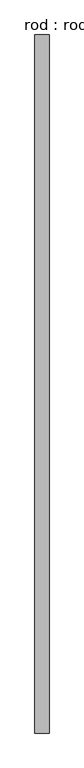
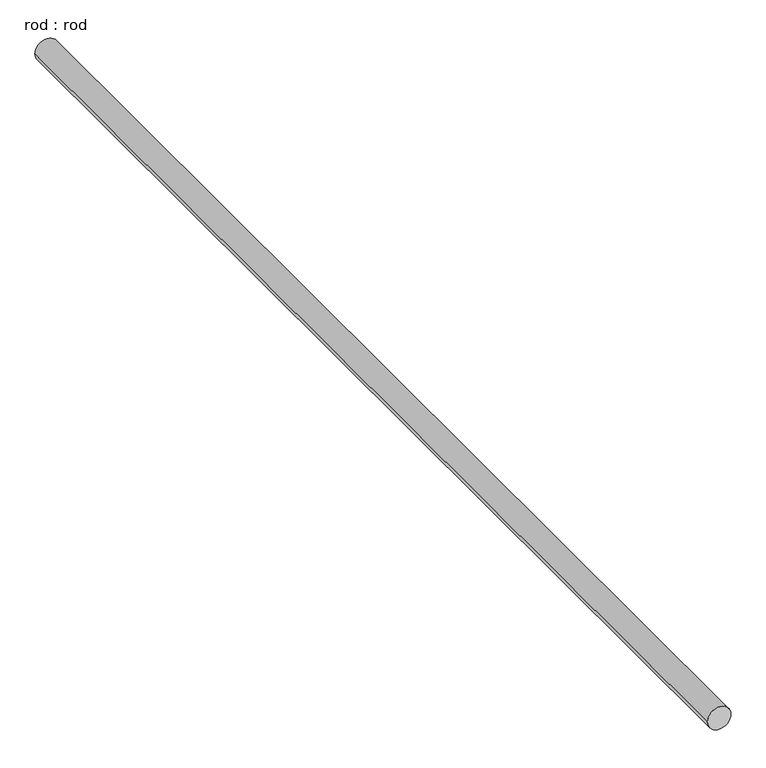
"""IFC4 building model written with IfcOpenShell, lengths in millimetres: proxy geometry, rod : rod."""

from ifc_helpers import new_model, si_unit, point, frame, frame_2d, origin, place, context, project, spatial, circle_curve, trimmed, segment, composite_curve, outline, extrude, source, transform, mapped, element, save


def rod_rod_c0665fd1(model_context):
    return source(origin(), model_context, "Body", "SweptSolid", [
        extrude(outline(composite_curve([segment(trimmed(circle_curve(frame_2d((0.0108462, 0.0)), 200.0), [point((0.0108462, 200.0))], [point((0.0108462, -200.0))], False, "CARTESIAN"), True, "CONTINUOUS"), segment(trimmed(circle_curve(frame_2d((0.0108462, 0.0)), 200.0), [point((0.0108462, -200.0))], [point((0.0108462, 200.0))], False, "CARTESIAN"), True, "CONTINUOUS")], self_intersect=False)), frame((0.0, -5782.2713847, 0.0), z_axis=(0.0, 1.0, 0.0), x_axis=(0.0, 0.0, 1.0)), (0.0, 0.0, 1.0), 19750.0),
    ])


if __name__ == "__main__":
    model = new_model("IFC4")
    model_context = context("Model", 3, world=origin())
    ifc_project = project(units=[si_unit("LENGTHUNIT", "METRE", prefix="MILLI")], contexts=[model_context])
    site = spatial("IfcSite", under=ifc_project)
    building = spatial("IfcBuilding", under=site)
    placement = place(None, origin())
    rod_rod_shape = rod_rod_c0665fd1(model_context)
    element("IfcBuildingElementProxy", 1, Name="rod : rod", ObjectType="rod : rod", at=placement, inside=building, context=model_context, shape_type="MappedRepresentation", body=[
        mapped(rod_rod_shape, transform((0.0, 0.0, 0.0), x_axis=(1.0, 0.0, 0.0), y_axis=(0.0, 1.0, 0.0), z_axis=(0.0, 0.0, 1.0))),
    ])
    save(model, "model.ifc")

# Revit data of these elements
# Type "rod : rod"
#   Default Elevation = 0
